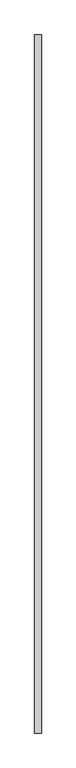
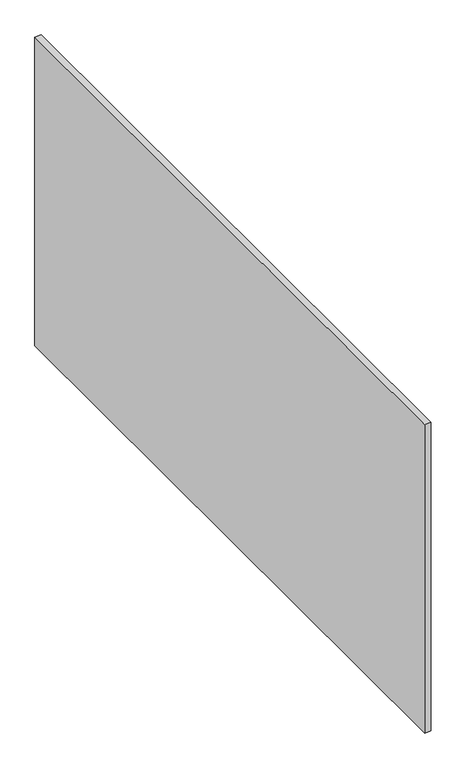
"""IFC4 building model written with IfcOpenShell, lengths in millimetres: proxy geometry, Plywood066 209 : Plywood066 209."""

from ifc_helpers import new_model, si_unit, frame, origin, place, context, project, spatial, polyline, outline, extrude, source, transform, mapped, element, save


def generic_models_5195f518(model_context):
    return source(origin(), model_context, "Body", "SweptSolid", [
        extrude(outline(polyline([(-9641.274441, 7982.1529359), (-9660.321316, 7982.1529359), (-9660.321316, 9982.1529359), (-9641.274441, 9982.1529359), (-9641.274441, 7982.1529359)])), frame((0.0, 0.0, 32568.8960253), z_axis=(0.0, 0.0, 1.0), x_axis=(1.0, 0.0, 0.0)), (0.0, 0.0, 1.0), 965.2),
    ])


if __name__ == "__main__":
    model = new_model("IFC4")
    model_context = context("Model", 3, world=origin())
    ifc_project = project(units=[si_unit("LENGTHUNIT", "METRE", prefix="MILLI")], contexts=[model_context])
    site = spatial("IfcSite", under=ifc_project)
    building = spatial("IfcBuilding", under=site)
    placement = place(None, origin())
    generic_models_shape = generic_models_5195f518(model_context)
    element("IfcBuildingElementProxy", 1, Name="Plywood066 209 : Plywood066 209", ObjectType="Plywood066 209 : Plywood066 209", at=placement, inside=building, context=model_context, shape_type="MappedRepresentation", body=[
        mapped(generic_models_shape, transform((0.0, 0.0, 0.0), x_axis=(1.0, 0.0, 0.0), y_axis=(0.0, 1.0, 0.0), z_axis=(0.0, 0.0, 1.0))),
    ])
    save(model, "model.ifc")

# Revit data of these elements
# Type "Plywood066 209 : Plywood066 209"
#   NameOverride = "Plywood066"
# Element 1 (IfcBuildingElementProxy, "Plywood066 209 : Plywood066 209")
#   Materials on its faces: "CDX PLYWOOD -  SEE STRUCTURAL DWGS"
# Materials
#   "CDX PLYWOOD -  SEE STRUCTURAL DWGS": class "Unassigned", colour RGB 177 130 114, transparency 0, Cost = 0
